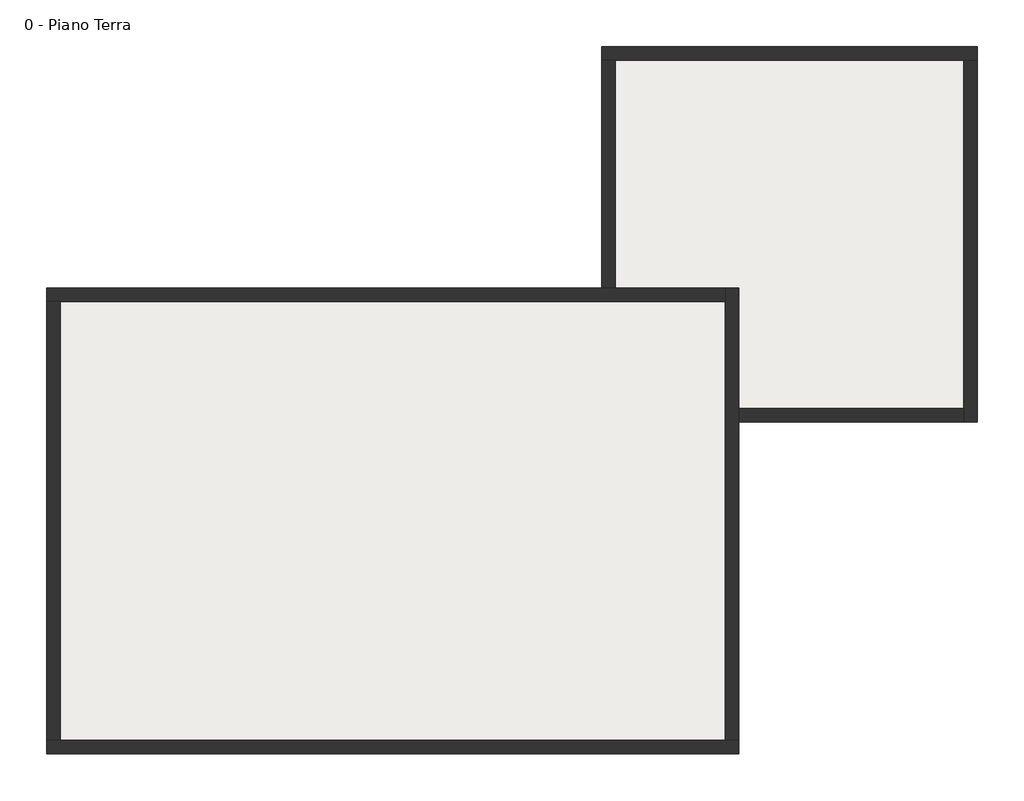
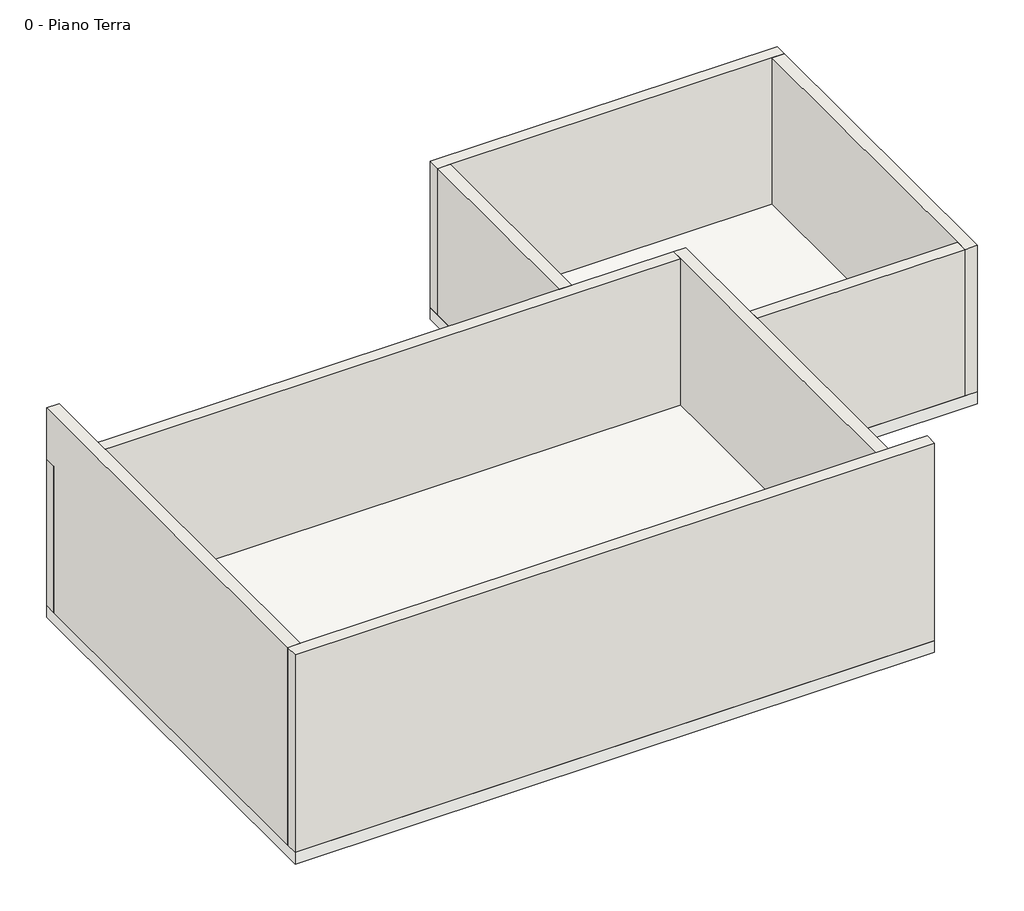
# One storey: 8 walls, 2 slabs.
"""IFC4 building model written with IfcOpenShell, lengths in millimetres."""

from ifc_helpers import new_model, si_unit, frame, origin, origin_with_axes, place, context, project, spatial, polyline, outline, extrude, faceted_brep, element, save

model = new_model("IFC4")

# Units and contexts
model_context = context("Model", 3, world=origin())
ifc_project = project(units=[si_unit("LENGTHUNIT", "METRE", prefix="MILLI")], contexts=[model_context])

# Site, building, storey
site = spatial("IfcSite", under=ifc_project)
building = spatial("IfcBuilding", under=site)
storey = spatial("IfcBuildingStorey", under=building, Name="0 - Piano Terra", Elevation=0.0)

# Slabs
placement = place(None, origin())
element("IfcSlab", 1, ObjectType="Latero Cementizio - 30 cm", at=placement, inside=storey, context=model_context, shape_type="SweptSolid", body=[
    extrude(outline(polyline([(-8493.3820144, 7328.6453385), (6806.6179856, 7328.6453385), (6806.6179856, -2971.3546615), (-8493.3820144, -2971.3546615), (-8493.3820144, 7328.6453385)])), frame((0.0, 0.0, -300.0), z_axis=(0.0, 0.0, 1.0), x_axis=(1.0, 0.0, 0.0)), (0.0, 0.0, 1.0), 300.0),
])
element("IfcSlab", 2, ObjectType="Latero Cementizio - 30 cm", at=placement, inside=storey, context=model_context, shape_type="SweptSolid", body=[
    extrude(outline(polyline([(6806.6179856, 4671.5492236), (6806.6179856, 7328.6453385), (4077.4891128, 7328.6453385), (3777.4891128, 7328.6453385), (3777.4891128, 12671.5492236), (12077.4891128, 12671.5492236), (12077.4891128, 4371.5492236), (6806.6179856, 4371.5492236), (6806.6179856, 4671.5492236)])), frame((0.0, 0.0, -300.0), z_axis=(0.0, 0.0, 1.0), x_axis=(1.0, 0.0, 0.0)), (0.0, 0.0, 1.0), 300.0),
])

# Walls
element("IfcWall", 3, ObjectType="Generico - 30 cm", at=placement, inside=storey, context=model_context, shape_type="Brep", body=[
    faceted_brep([(-8493.3820144, -2971.3546615, 0.0), (6806.6179856, -2971.3546615, 0.0), (6806.6179856, -2971.3546615, 5000.0), (-8493.3820144, -2971.3546615, 5000.0), (-8493.3820144, -2671.3546615, 0.0), (-8493.3820144, -2671.3546615, 5000.0), (-8193.3820144, -2671.3546615, 5000.0), (6506.6179856, -2671.3546615, 5000.0), (6806.6179856, -2671.3546615, 5000.0), (6806.6179856, -2671.3546615, 3700.0), (6806.6179856, -2671.3546615, 0.0), (6506.6179856, -2671.3546615, 0.0), (-8193.3820144, -2671.3546615, 0.0)], [[[0, 1, 2, 3]], [[4, 5, 6, 7, 8, 9, 10, 11, 12]], [[1, 0, 4, 12, 11, 10]], [[3, 2, 8, 7, 6, 5]], [[0, 3, 5, 4]], [[1, 10, 9, 8, 2]]]),
])
element("IfcWall", 4, ObjectType="Generico - 30 cm", at=placement, inside=storey, context=model_context, shape_type="Brep", body=[
    faceted_brep([(6806.6179856, -2671.3546615, 0.0), (6806.6179856, 4371.5492236, 0.0), (6806.6179856, 4671.5492236, 0.0), (6806.6179856, 7328.6453385, 0.0), (6806.6179856, 7328.6453385, 3700.0), (6806.6179856, 4671.5492236, 3700.0), (6806.6179856, 4371.5492236, 3700.0), (6806.6179856, 2871.5492236, 3700.0), (6806.6179856, -2671.3546615, 3700.0), (6506.6179856, -2671.3546615, 0.0), (6506.6179856, -2671.3546615, 3700.0), (6506.6179856, 2871.5492236, 3700.0), (6506.6179856, 7028.6453385, 3700.0), (6506.6179856, 7328.6453385, 3700.0), (6506.6179856, 7328.6453385, 0.0), (6506.6179856, 7028.6453385, 0.0)], [[[0, 1, 2, 3, 4, 5, 6, 7, 8]], [[9, 10, 11, 12, 13, 14, 15]], [[3, 2, 1, 0, 9, 15, 14]], [[8, 7, 6, 5, 4, 13, 12, 11, 10]], [[4, 3, 14, 13]], [[0, 8, 10, 9]]]),
])
element("IfcWall", 5, ObjectType="Generico - 30 cm", at=placement, inside=storey, context=model_context, shape_type="Brep", body=[
    faceted_brep([(6506.6179856, 7328.6453385, 0.0), (4077.4891128, 7328.6453385, 0.0), (3777.4891128, 7328.6453385, 0.0), (-8493.3820144, 7328.6453385, 0.0), (-8493.3820144, 7328.6453385, 3700.0), (-8193.3820144, 7328.6453385, 3700.0), (2277.4891128, 7328.6453385, 3700.0), (3777.4891128, 7328.6453385, 3700.0), (4077.4891128, 7328.6453385, 3700.0), (6506.6179856, 7328.6453385, 3700.0), (6506.6179856, 7028.6453385, 0.0), (6506.6179856, 7028.6453385, 3700.0), (2277.4891128, 7028.6453385, 3700.0), (-8193.3820144, 7028.6453385, 3700.0), (-8493.3820144, 7028.6453385, 3700.0), (-8493.3820144, 7028.6453385, 0.0), (-8193.3820144, 7028.6453385, 0.0)], [[[0, 1, 2, 3, 4, 5, 6, 7, 8, 9]], [[10, 11, 12, 13, 14, 15, 16]], [[3, 2, 1, 0, 10, 16, 15]], [[9, 8, 7, 6, 5, 4, 14, 13, 12, 11]], [[4, 3, 15, 14]], [[0, 9, 11, 10]]]),
])
element("IfcWall", 6, ObjectType="Generico - 30 cm", at=placement, inside=storey, context=model_context, shape_type="Brep", body=[
    faceted_brep([(-8493.3820144, 7028.6453385, 0.0), (-8493.3820144, -2671.3546615, 0.0), (-8493.3820144, -2671.3546615, 5000.0), (-8493.3820144, 7328.6453385, 5000.0), (-8493.3820144, 7328.6453385, 3700.0), (-8493.3820144, 7028.6453385, 3700.0), (-8193.3820144, 7028.6453385, 0.0), (-8193.3820144, 7028.6453385, 3700.0), (-8193.3820144, 7328.6453385, 3700.0), (-8193.3820144, 7328.6453385, 5000.0), (-8193.3820144, 7028.6453385, 5000.0), (-8193.3820144, -2671.3546615, 5000.0), (-8193.3820144, -2671.3546615, 0.0)], [[[0, 1, 2, 3, 4, 5]], [[6, 7, 8, 9, 10, 11, 12]], [[1, 0, 6, 12]], [[3, 2, 11, 10, 9]], [[2, 1, 12, 11]], [[4, 8, 7, 5]], [[0, 5, 7, 6]], [[4, 3, 9, 8]]]),
])
element("IfcWall", 7, ObjectType="Generico - 30 cm", at=placement, inside=storey, context=model_context, shape_type="Brep", body=[
    faceted_brep([(3777.4891128, 12371.5492236, 0.0), (4077.4891128, 12371.5492236, 0.0), (11777.4891128, 12371.5492236, 0.0), (12077.4891128, 12371.5492236, 0.0), (12077.4891128, 12371.5492236, 3700.0), (11777.4891128, 12371.5492236, 3700.0), (4077.4891128, 12371.5492236, 3700.0), (3777.4891128, 12371.5492236, 3700.0), (3777.4891128, 12671.5492236, 0.0), (3777.4891128, 12671.5492236, 3700.0), (12077.4891128, 12671.5492236, 3700.0), (12077.4891128, 12671.5492236, 0.0)], [[[0, 1, 2, 3, 4, 5, 6, 7]], [[8, 9, 10, 11]], [[3, 2, 1, 0, 8, 11]], [[7, 6, 5, 4, 10, 9]], [[4, 3, 11, 10]], [[0, 7, 9, 8]]]),
])
element("IfcWall", 8, ObjectType="Generico - 30 cm", at=placement, inside=storey, context=model_context, shape_type="Brep", body=[
    faceted_brep([(11777.4891128, 12371.5492236, 0.0), (11777.4891128, 4671.5492236, 0.0), (11777.4891128, 4371.5492236, 0.0), (11777.4891128, 4371.5492236, 3700.0), (11777.4891128, 4671.5492236, 3700.0), (11777.4891128, 12371.5492236, 3700.0), (12077.4891128, 12371.5492236, 0.0), (12077.4891128, 12371.5492236, 3700.0), (12077.4891128, 4371.5492236, 3700.0), (12077.4891128, 4371.5492236, 0.0)], [[[0, 1, 2, 3, 4, 5]], [[6, 7, 8, 9]], [[2, 1, 0, 6, 9]], [[5, 4, 3, 8, 7]], [[0, 5, 7, 6]], [[3, 2, 9, 8]]]),
])
element("IfcWall", 9, ObjectType="Generico - 30 cm", at=placement, inside=storey, context=model_context, shape_type="SweptSolid", body=[
    extrude(outline(polyline([(6806.6179856, 4671.5492236), (11777.4891128, 4671.5492236), (11777.4891128, 4371.5492236), (6806.6179856, 4371.5492236), (6806.6179856, 4671.5492236)])), origin_with_axes(), (0.0, 0.0, 1.0), 3700.0),
])
element("IfcWall", 10, ObjectType="Generico - 30 cm", at=placement, inside=storey, context=model_context, shape_type="SweptSolid", body=[
    extrude(outline(polyline([(4077.4891128, 12371.5492236), (4077.4891128, 7328.6453385), (3777.4891128, 7328.6453385), (3777.4891128, 12371.5492236), (4077.4891128, 12371.5492236)])), origin_with_axes(), (0.0, 0.0, 1.0), 3700.0),
])

save(model, "model.ifc")

# Revit data of these elements
# Project information
#   Data di consegna del progetto = "Data"
#   Stato del progetto = "Stato"
#   Nome del cliente = "Proprietario"
#   Nome del progetto = "Nome"
#   Numero del progetto = "0001"
# Type "Latero Cementizio - 30 cm"
#   Keynote = "S/3"
#   Function = 0
#   Layers, outside or top first: 0.02 m "Ceramica bianca" (function 4); 0.065 m "Sabbia e Calcestruzzo" (function 2); 0.04 m "Calcestruzzo" (function 1); 0.16 m "Laterizio (2)" (function 1); 0.015 m "Intonaco - Bianco" (function 5)
# Type "Generico - 30 cm"
#   Keynote = "Mb/3"
#   Layers, outside or top first: 0.30 m "Default - Muro" (function 1)
# Element 1 (IfcSlab, "Latero Cementizio - 30 cm")
#   built-in parameter 1001955 = 3.14159 (stored number, unit not read)
#   Height Offset From Level = 0.00 m
#   built-in parameter 1001954 = 1
#   Phase Created = Stato di Progetto
#   Materials on its faces: "Intonaco - Bianco", "Ceramica bianca"
# Element 2 (IfcSlab, "Latero Cementizio - 30 cm")
#   built-in parameter 1001955 = 1.5708 (stored number, unit not read)
#   Height Offset From Level = 0.00 m
#   Phase Created = Stato di Progetto
#   Materials on its faces: "Intonaco - Bianco", "Ceramica bianca"
# Elements 3, 6 (IfcWall, "Generico - 30 cm")
#   Top Offset = 0.00 m
#   Base Offset = 0.00 m
#   Unconnected Height = 5.00 m
#   wall height = 5.00 m
#   Phase Created = Stato di Progetto
#   Base Constraint = 0 - Piano Terra
#   Materials on its faces: "Default - Muro"
# Elements 4, 5, 7, 8, 9, 10 (IfcWall, "Generico - 30 cm")
#   Top Offset = 0.00 m
#   Base Offset = 0.00 m
#   Unconnected Height = 3.70 m
#   wall height = 3.70 m
#   Phase Created = Stato di Progetto
#   Base Constraint = 0 - Piano Terra
#   Materials on its faces: "Default - Muro"
# Materials
#   "Ceramica bianca": class "Ceramica", colour RGB 210 210 210, transparency 0, Description = "Finitura interna - Piastrelle di ceramica incollate", Cost = 0
#   "Sabbia e Calcestruzzo": class "Calcestruzzo", colour RGB 127 127 127, transparency 0, Description = "Magrone - Sabbia e cemento", Cost = 0
#   "Calcestruzzo": class "Calcestruzzo", colour RGB 192 192 192, transparency 0, Description = "Calcestruzzo - Cemento Portland", Cost = 0
#   "Laterizio (2)": class "Mattone", colour RGB 255 128 64, transparency 0, Description = "Pignatta h 16 cm", Cost = 0
#   "Intonaco - Bianco": class "Intonaco", colour RGB 249 249 249, transparency 0, Description = "Verniciatura", Cost = 0
#   "Default - Muro": class "Varie", colour RGB 127 127 127, transparency 0, Cost = 0
